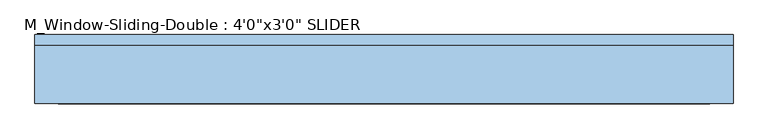
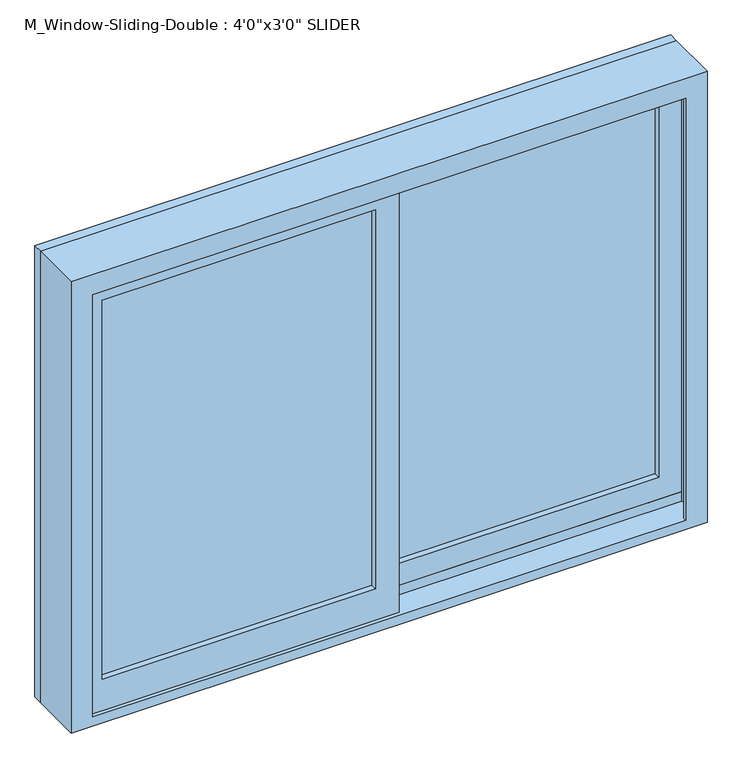
"""IFC4 building model written with IfcOpenShell, lengths in millimetres: window geometry."""

from ifc_helpers import new_model, si_unit, frame, origin, place, context, project, spatial, polyline, outline, extrude, faceted_brep, source, transform, mapped, element, save


def window_a3b47c69(model_context):
    return source(origin(), model_context, "Body", "SolidModel", [
        faceted_brep([(-609.6, 35.56, 900.0), (609.6, 35.56, 900.0), (609.6, -66.04, 900.0), (-609.6, -66.04, 900.0), (-568.6778905, -66.04, 1773.4778905), (-568.6778905, -66.04, 919.05), (-568.6778905, -59.69, 919.05), (-568.6778905, -59.69, 1773.4778905), (-590.55, -59.69, 919.05), (-590.55, -59.69, 1795.35), (590.55, -59.69, 1795.35), (590.55, -59.69, 919.05), (568.6778905, -59.69, 919.05), (568.6778905, -59.69, 1773.4778905), (-590.55, -15.24, 919.05), (-590.55, -15.24, 938.1), (-590.55, 29.21, 938.1), (-590.55, 29.21, 919.05), (-590.55, 35.56, 919.05), (-590.55, 35.56, 1795.35), (-609.6, 35.56, 1814.4), (609.6, 35.56, 1814.4), (590.55, 35.56, 1795.35), (590.55, 35.56, 919.05), (-609.6, -66.04, 1814.4), (609.6, -66.04, 1814.4), (568.6778905, -66.04, 1773.4778905), (568.6778905, -66.04, 919.05), (590.55, 29.21, 919.05), (590.55, 29.21, 938.1), (590.55, -15.24, 938.1), (590.55, -15.24, 919.05)], [[[0, 1, 2, 3]], [[4, 5, 6, 7]], [[7, 6, 8, 9, 10, 11, 12, 13]], [[9, 8, 14, 15, 16, 17, 18, 19]], [[0, 20, 21, 1], [22, 19, 18, 23]], [[24, 20, 0, 3]], [[2, 25, 24, 3], [4, 26, 27, 5]], [[7, 13, 26, 4]], [[9, 19, 22, 10]], [[20, 24, 25, 21]], [[13, 12, 27, 26]], [[22, 23, 28, 29, 30, 31, 11, 10]], [[21, 25, 2, 1]], [[27, 12, 11, 31, 14, 8, 6, 5]], [[31, 30, 15, 14]], [[30, 29, 16, 15]], [[29, 28, 17, 16]], [[18, 17, 28, 23]]]),
        extrude(outline(polyline([(1814.4, 609.6), (1814.4, -609.6), (900.0, -609.6), (900.0, 609.6), (1814.4, 609.6)]), holes=[polyline([(1795.35, -590.55), (1795.35, 590.55), (919.05, 590.55), (919.05, -590.55), (1795.35, -590.55)])]), frame((0.0, 35.56, 0.0), z_axis=(0.0, 1.0, 0.0), x_axis=(0.0, 0.0, 1.0)), (0.0, 0.0, 1.0), 19.05),
        extrude(outline(polyline([(546.1, -2.54), (22.225, -2.54), (22.225, 3.81), (546.1, 3.81), (546.1, -2.54)])), frame((0.0, 0.0, 982.55), z_axis=(0.0, 0.0, 1.0), x_axis=(1.0, 0.0, 0.0)), (0.0, 0.0, 1.0), 768.35),
        extrude(outline(polyline([(546.1, 10.16), (22.225, 10.16), (22.225, 16.51), (546.1, 16.51), (546.1, 10.16)])), frame((0.0, 0.0, 982.55), z_axis=(0.0, 0.0, 1.0), x_axis=(1.0, 0.0, 0.0)), (0.0, 0.0, 1.0), 768.35),
        extrude(outline(polyline([(-22.225, -46.99), (-546.1, -46.99), (-546.1, -40.64), (-22.225, -40.64), (-22.225, -46.99)])), frame((0.0, 0.0, 982.55), z_axis=(0.0, 0.0, 1.0), x_axis=(1.0, 0.0, 0.0)), (0.0, 0.0, 1.0), 768.35),
        extrude(outline(polyline([(-22.225, -34.29), (-546.1, -34.29), (-546.1, -27.94), (-22.225, -27.94), (-22.225, -34.29)])), frame((0.0, 0.0, 982.55), z_axis=(0.0, 0.0, 1.0), x_axis=(1.0, 0.0, 0.0)), (0.0, 0.0, 1.0), 768.35),
        extrude(outline(polyline([(919.05, 22.225), (1795.35, 22.225), (1795.35, -590.55), (919.05, -590.55), (919.05, 22.225)]), holes=[polyline([(1750.9, -546.1), (1750.9, -22.225), (982.55, -22.225), (982.55, -546.1), (1750.9, -546.1)])]), frame((0.0, -59.69, 0.0), z_axis=(0.0, 1.0, 0.0), x_axis=(0.0, 0.0, 1.0)), (0.0, 0.0, 1.0), 44.45),
        extrude(outline(polyline([(938.1, -22.225), (938.1, 590.55), (1795.35, 590.55), (1795.35, -22.225), (938.1, -22.225)]), holes=[polyline([(982.55, 546.1), (982.55, 22.225), (1750.9, 22.225), (1750.9, 546.1), (982.55, 546.1)])]), frame((0.0, -15.24, 0.0), z_axis=(0.0, 1.0, 0.0), x_axis=(0.0, 0.0, 1.0)), (0.0, 0.0, 1.0), 44.45),
    ])


if __name__ == "__main__":
    model = new_model("IFC4")
    model_context = context("Model", 3, world=origin())
    ifc_project = project(units=[si_unit("LENGTHUNIT", "METRE", prefix="MILLI")], contexts=[model_context])
    site = spatial("IfcSite", under=ifc_project)
    building = spatial("IfcBuilding", under=site)
    placement = place(None, origin())
    window_shape = window_a3b47c69(model_context)
    element("IfcWindow", 1, ObjectType="M_Window-Sliding-Double : 4'0\"x3'0\" SLIDER", at=placement, inside=building, context=model_context, shape_type="MappedRepresentation", body=[
        mapped(window_shape, transform((0.0, 0.0, 0.0), x_axis=(1.0, 0.0, 0.0), y_axis=(0.0, 1.0, 0.0), z_axis=(0.0, 0.0, 1.0))),
    ])
    save(model, "model.ifc")

# Revit data of these elements
# Type "M_Window-Sliding-Double : 4'0\"x3'0\" SLIDER"
#   Type Mark = "3"
#   Fire Rating = "0.5h"
#   Assembly Code = "B2020100"
#   Analytic Construction = "Double glazing - domestic"
#   Window Inset [instance default] = 0' - 0"
#   Wall Thickness [instance default] = 0' - 5.90551"
#   Visual Light Transmittance = 0.81
#   Thermal Resistance (R) = 1.8146 (h·ft²·°F)/BTU
#   Solar Heat Gain Coefficient = 0.76
#   Muntin Width = 1' - 8 5/8"
#   Muntin Height = 2' - 6 1/4"
#   Interior Wall Closure [instance default] = 0' - 2.65551"
#   Heat Transfer Coefficient (U) = 0.5511 BTU/(h·ft²·°F)
#   Frame Extension [instance default] = 0' - 0 1/4"
#   Exterior Wall Closure [instance default] = 0' - 1 1/4"
#   Rough Width = 4' - 0.59055"
#   Rough Height = 3' - 0.59055"
#   Height = 3' - 0"
#   Extension Jamb [instance default] = 0' - 2.65551"
#   Default Sill Height = 2' - 11.43307"
#   Width = 4' - 0"
#   Interior Trim Visibility [instance default] = yes
#   Indicator Visibility [instance default] = yes
#   Exterior Trim Visibility [instance default] = yes
#   Muntin Visibility = yes
#   Extension Jamb Visibility [instance default] = yes
#   Muntin Pattern = M_Muntin Pattern_2x2 : M_Muntin Pattern_2x2
#   Interior Trim Material = Wood - Stained
#   Interior Trim = M_Trim-Window-Interior-Flat : Picture Frame
#   Interior Frame Material = Wood - Stained
#   Glass Panel Material = Glass
#   Exterior Trim Material = Clad - White
#   Exterior Trim = M_Trim-Window-Exterior-Flat : with Sill
#   Exterior Frame Material = Clad - White
#   Wall Closure = (empty or 0)
# Element 1 (IfcWindow, "M_Window-Sliding-Double : 4'0\"x3'0\" SLIDER")
#   Wall Thickness = 0' - 4"
#   Extension Jamb = 0' - 0 3/4"
#   Materials on its faces: "Wood - Stained", "Glass", "Clad - White"
# Materials
#   "Wood - Stained": class "Wood", colour RGB 224 178 126, transparency 0, Cost = 0
#   "Glass": class "Glass", colour RGB 0 128 192, transparency 0.75, Description = "Soda Lime Glass", Cost = 0
#   "Clad - White": class "Wood", colour RGB 242 242 238, transparency 0, Cost = 0
